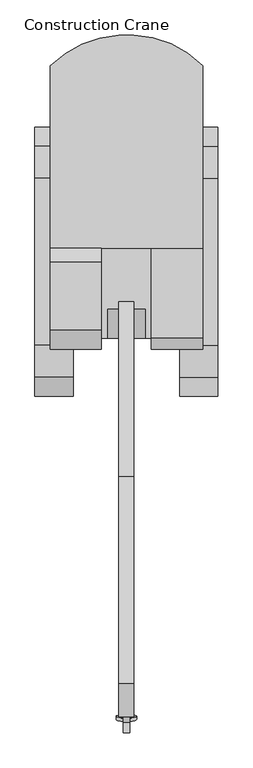
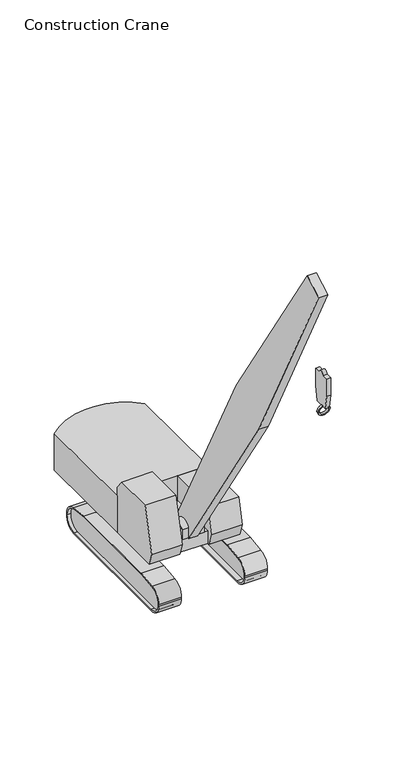
"""IFC4 building model written with IfcOpenShell, lengths in millimetres: geographic element geometry, Construction Crane : 50' @ 60 deg."""

from ifc_helpers import new_model, si_unit, point, frame, frame_2d, origin, place, context, project, spatial, polyline, circle_curve, trimmed, segment, composite_curve, outline, extrude, source, transform, mapped, element, save


def construction_crane_787d4a5c(model_context):
    return source(origin(), model_context, "Body", "SweptSolid", [
        extrude(outline(composite_curve([segment(polyline([(-4575.608491, 934.26875), (-1239.0684321, 934.26875), (-625.3121051, 856.1386871)]), True, "CONTINUOUS"), segment(trimmed(circle_curve(frame_2d((-676.8331731, 453.3411993)), 406.0791014), [point((-625.3121051, 856.1386871))], [point((-270.7700765, 456.946505))], False, "CARTESIAN"), True, "CONTINUOUS"), segment(trimmed(circle_curve(frame_2d((-676.7161092, 456.946505)), 405.9460328), [point((-270.7700765, 456.946505))], [point((-676.7161092, 51.0004722))], False, "CARTESIAN"), True, "CONTINUOUS"), segment(polyline([(-676.7161092, 51.0004722), (-5143.9371049, 51.0004722)]), True, "CONTINUOUS"), segment(trimmed(circle_curve(frame_2d((-5143.9371049, 451.7022639)), 400.7017917), [point((-5143.9371049, 51.0004722))], [point((-5544.6388966, 451.7022639))], False, "CARTESIAN"), True, "CONTINUOUS"), segment(trimmed(circle_curve(frame_2d((-5137.6945084, 451.7710081)), 406.944394), [point((-5544.6388966, 451.7022639))], [point((-5189.1160735, 855.4535101))], False, "CARTESIAN"), True, "CONTINUOUS"), segment(polyline([(-5189.1160735, 855.4535101), (-4575.608491, 934.26875)]), True, "CONTINUOUS")], self_intersect=False)), frame((-4426.6809216, 0.0, 0.0), z_axis=(1.0, 0.0, 0.0), x_axis=(0.0, 1.0, 0.0)), (0.0, 0.0, 1.0), 464.6393791),
        extrude(outline(composite_curve([segment(polyline([(-651.6384615, 0.0), (-5163.0384615, 0.0)]), True, "CONTINUOUS"), segment(trimmed(circle_curve(frame_2d((-5163.0384615, 431.8)), 431.8), [point((-5163.0384615, 0.0))], [point((-5594.8384615, 431.8))], False, "CARTESIAN"), True, "CONTINUOUS"), segment(polyline([(-5594.8384615, 431.8), (-5594.8384615, 475.1036968)]), True, "CONTINUOUS"), segment(trimmed(circle_curve(frame_2d((-5163.0384615, 475.1036968)), 431.8), [point((-5594.8384615, 475.1036968))], [point((-5217.7268735, 903.4264928))], False, "CARTESIAN"), True, "CONTINUOUS"), segment(polyline([(-5217.7268735, 903.4264928), (-4578.8384615, 985.06875), (-1235.8384615, 985.06875), (-596.9500496, 903.4264928)]), True, "CONTINUOUS"), segment(trimmed(circle_curve(frame_2d((-651.6384615, 475.1036968)), 431.8), [point((-596.9500496, 903.4264928))], [point((-219.8384615, 475.1036968))], False, "CARTESIAN"), True, "CONTINUOUS"), segment(polyline([(-219.8384615, 475.1036968), (-219.8384615, 431.8)]), True, "CONTINUOUS"), segment(trimmed(circle_curve(frame_2d((-651.6384615, 431.8)), 431.8), [point((-219.8384615, 431.8))], [point((-651.6384615, 0.0))], False, "CARTESIAN"), True, "CONTINUOUS")], self_intersect=False), holes=[composite_curve([segment(polyline([(-4575.608491, 934.26875), (-5189.1160735, 855.3847601)]), True, "CONTINUOUS"), segment(trimmed(circle_curve(frame_2d((-5137.6945084, 451.7022639)), 406.9443882), [point((-5189.1160735, 855.3847601))], [point((-5544.6388966, 451.7022639))], True, "CARTESIAN"), True, "CONTINUOUS"), segment(trimmed(circle_curve(frame_2d((-5143.9371049, 451.7022639)), 400.7017917), [point((-5544.6388966, 451.7022639))], [point((-5143.9371049, 51.0004722))], True, "CARTESIAN"), True, "CONTINUOUS"), segment(polyline([(-5143.9371049, 51.0004722), (-676.7161092, 51.0004722)]), True, "CONTINUOUS"), segment(trimmed(circle_curve(frame_2d((-676.7161092, 456.946505)), 405.9460328), [point((-676.7161092, 51.0004722))], [point((-270.7700765, 456.946505))], True, "CARTESIAN"), True, "CONTINUOUS"), segment(trimmed(circle_curve(frame_2d((-676.8331731, 453.2718224)), 406.0797233), [point((-270.7700765, 456.946505))], [point((-625.3121051, 856.0699371))], True, "CARTESIAN"), True, "CONTINUOUS"), segment(polyline([(-625.3121051, 856.0699371), (-1239.0684321, 934.26875), (-4575.608491, 934.26875)]), True, "CONTINUOUS")], self_intersect=False)]), frame((-4612.32123, 0.0, 0.0), z_axis=(1.0, 0.0, 0.0), x_axis=(0.0, 1.0, 0.0)), (0.0, 0.0, 1.0), 762.0),
        extrude(outline(composite_curve([segment(polyline([(-4575.608491, 934.26875), (-1239.0684321, 934.26875), (-625.3121051, 856.1386871)]), True, "CONTINUOUS"), segment(trimmed(circle_curve(frame_2d((-676.8331731, 453.3411993)), 406.0791014), [point((-625.3121051, 856.1386871))], [point((-270.7700765, 456.946505))], False, "CARTESIAN"), True, "CONTINUOUS"), segment(trimmed(circle_curve(frame_2d((-676.7161092, 456.946505)), 405.9460328), [point((-270.7700765, 456.946505))], [point((-676.7161092, 51.0004722))], False, "CARTESIAN"), True, "CONTINUOUS"), segment(polyline([(-676.7161092, 51.0004722), (-5143.9005487, 51.0004722)]), True, "CONTINUOUS"), segment(trimmed(circle_curve(frame_2d((-5143.9005487, 451.7388201)), 400.738348), [point((-5143.9005487, 51.0004722))], [point((-5544.6388966, 451.7388201))], False, "CARTESIAN"), True, "CONTINUOUS"), segment(trimmed(circle_curve(frame_2d((-5137.6579522, 451.7388201)), 406.9809445), [point((-5544.6388966, 451.7388201))], [point((-5189.1160735, 855.4535101))], False, "CARTESIAN"), True, "CONTINUOUS"), segment(polyline([(-5189.1160735, 855.4535101), (-4575.608491, 934.26875)]), True, "CONTINUOUS")], self_intersect=False)), frame((-7396.2009175, 0.0, 0.0), z_axis=(1.0, 0.0, 0.0), x_axis=(0.0, 1.0, 0.0)), (0.0, 0.0, 1.0), 464.6393791),
        extrude(outline(composite_curve([segment(polyline([(-3855.5873985, 1944.8065119), (-3855.5873985, 1589.2065119), (-4435.4967838, 1589.2065119), (-4435.4967838, 1944.8065119)]), True, "CONTINUOUS"), segment(trimmed(circle_curve(frame_2d((-4145.5420911, 1746.7297499)), 351.15257), [point((-4435.4967838, 1944.8065119))], [point((-3855.5873985, 1944.8065119))], False, "CARTESIAN"), True, "CONTINUOUS")], self_intersect=False)), frame((-6056.08998, 0.0, 0.0), z_axis=(1.0, 0.0, 0.0), x_axis=(0.0, 1.0, 0.0)), (0.0, 0.0, 1.0), 755.1034902),
        extrude(outline(polyline([(-5179.12123, -2642.3288049), (-5179.12123, -4433.7384615), (-6179.12123, -4433.7384615), (-6179.12123, -2642.3288049), (-5179.12123, -2642.3288049)])), frame((0.0, 0.0, 1155.0), z_axis=(0.0, 0.0, 1.0), x_axis=(1.0, 0.0, 0.0)), (0.0, 0.0, 1.0), 434.1377619),
        extrude(outline(composite_curve([segment(polyline([(-651.6384615, 0.0), (-5163.0384615, 0.0)]), True, "CONTINUOUS"), segment(trimmed(circle_curve(frame_2d((-5163.0384615, 431.8)), 431.8), [point((-5163.0384615, 0.0))], [point((-5594.8384615, 431.8))], False, "CARTESIAN"), True, "CONTINUOUS"), segment(polyline([(-5594.8384615, 431.8), (-5594.8384615, 475.1036968)]), True, "CONTINUOUS"), segment(trimmed(circle_curve(frame_2d((-5163.0384615, 475.1036968)), 431.8), [point((-5594.8384615, 475.1036968))], [point((-5217.7268735, 903.4264928))], False, "CARTESIAN"), True, "CONTINUOUS"), segment(polyline([(-5217.7268735, 903.4264928), (-4578.8384615, 985.06875), (-1235.8384615, 985.06875), (-596.9500496, 903.4264928)]), True, "CONTINUOUS"), segment(trimmed(circle_curve(frame_2d((-651.6384615, 475.1036968)), 431.8), [point((-596.9500496, 903.4264928))], [point((-219.8384615, 475.1036968))], False, "CARTESIAN"), True, "CONTINUOUS"), segment(polyline([(-219.8384615, 475.1036968), (-219.8384615, 431.8)]), True, "CONTINUOUS"), segment(trimmed(circle_curve(frame_2d((-651.6384615, 431.8)), 431.8), [point((-219.8384615, 431.8))], [point((-651.6384615, 0.0))], False, "CARTESIAN"), True, "CONTINUOUS")], self_intersect=False), holes=[composite_curve([segment(polyline([(-4575.608491, 934.26875), (-5189.1160735, 855.3847601)]), True, "CONTINUOUS"), segment(trimmed(circle_curve(frame_2d((-5137.6945084, 451.7022639)), 406.9443882), [point((-5189.1160735, 855.3847601))], [point((-5544.6388966, 451.7022639))], True, "CARTESIAN"), True, "CONTINUOUS"), segment(trimmed(circle_curve(frame_2d((-5143.9371049, 451.7022639)), 400.7017917), [point((-5544.6388966, 451.7022639))], [point((-5143.9371049, 51.0004722))], True, "CARTESIAN"), True, "CONTINUOUS"), segment(polyline([(-5143.9371049, 51.0004722), (-676.7161092, 51.0004722)]), True, "CONTINUOUS"), segment(trimmed(circle_curve(frame_2d((-676.7161092, 456.946505)), 405.9460328), [point((-676.7161092, 51.0004722))], [point((-270.7700765, 456.946505))], True, "CARTESIAN"), True, "CONTINUOUS"), segment(trimmed(circle_curve(frame_2d((-676.8331731, 453.2718224)), 406.0797233), [point((-270.7700765, 456.946505))], [point((-625.3121051, 856.0699371))], True, "CARTESIAN"), True, "CONTINUOUS"), segment(polyline([(-625.3121051, 856.0699371), (-1239.0684321, 934.26875), (-4575.608491, 934.26875)]), True, "CONTINUOUS")], self_intersect=False)]), frame((-7507.92123, 0.0, 0.0), z_axis=(1.0, 0.0, 0.0), x_axis=(0.0, 1.0, 0.0)), (0.0, 0.0, 1.0), 762.0),
        extrude(outline(composite_curve([segment(polyline([(-7203.12123, -2642.3288049), (-7203.12123, 1015.2711951)]), True, "CONTINUOUS"), segment(trimmed(circle_curve(frame_2d((-5666.4440826, -594.4023865)), 2225.4046136), [point((-7203.12123, 1015.2711951))], [point((-5831.52123, 1624.8711951))], False, "CARTESIAN"), True, "CONTINUOUS"), segment(polyline([(-5831.52123, 1624.8711951), (-5526.72123, 1624.8711951)]), True, "CONTINUOUS"), segment(trimmed(circle_curve(frame_2d((-5627.7327269, -450.2546729)), 2077.5828962), [point((-5526.72123, 1624.8711951))], [point((-4155.12123, 1015.2711951))], False, "CARTESIAN"), True, "CONTINUOUS"), segment(polyline([(-4155.12123, 1015.2711951), (-4155.12123, -2642.3288049), (-7203.12123, -2642.3288049)]), True, "CONTINUOUS")], self_intersect=False)), frame((0.0, 0.0, 1155.0), z_axis=(0.0, 0.0, 1.0), x_axis=(1.0, 0.0, 0.0)), (0.0, 0.0, 1.0), 1300.06875),
        extrude(outline(polyline([(-2642.3288049, 1155.06875), (-4509.1429639, 1155.06875), (-4662.3384615, 1584.1295061), (-4443.5105446, 2455.06875), (-2642.3288049, 2455.06875), (-2642.3288049, 1155.06875)])), frame((-5179.12123, 0.0, 0.0), z_axis=(1.0, 0.0, 0.0), x_axis=(0.0, 1.0, 0.0)), (0.0, 0.0, 1.0), 1024.0),
        extrude(outline(polyline([(-2642.3288049, 2759.86875), (-2642.3288049, 2455.06875), (-2642.3288049, 1155.06875), (-4509.1429639, 1155.06875), (-4662.3384615, 1584.1295061), (-4278.9384615, 3110.06875), (-2907.3384615, 3110.06875), (-2642.3288049, 2759.86875)])), frame((-7203.12123, 0.0, 0.0), z_axis=(1.0, 0.0, 0.0), x_axis=(0.0, 1.0, 0.0)), (0.0, 0.0, 1.0), 1024.0),
        extrude(outline(polyline([(-7211.0827225, 8686.8431812), (-3709.0413561, 1909.9296043), (-4412.9468043, 1503.5296043), (-8530.9054378, 7924.8431812), (-12010.949759, 14714.456758), (-11351.0384013, 15095.456758), (-7211.0827225, 8686.8431812)])), frame((-5831.52123, 0.0, 0.0), z_axis=(1.0, 0.0, 0.0), x_axis=(0.0, 1.0, 0.0)), (0.0, 0.0, 1.0), 304.8),
        extrude(outline(composite_curve([segment(trimmed(circle_curve(frame_2d((0.0, -203.2)), 203.2), [point((0.0, -406.4))], [point((0.0, 0.0))], False, "CARTESIAN"), True, "CONTINUOUS"), segment(trimmed(circle_curve(frame_2d((0.0, -203.2)), 203.2), [point((0.0, 0.0))], [point((0.0, -406.4))], False, "CARTESIAN"), True, "CONTINUOUS")], self_intersect=False), holes=[composite_curve([segment(trimmed(circle_curve(frame_2d((0.0, -203.2)), 152.4), [point((0.0, -355.6))], [point((0.0, -50.8))], True, "CARTESIAN"), True, "CONTINUOUS"), segment(trimmed(circle_curve(frame_2d((0.0, -203.2)), 152.4), [point((0.0, -50.8))], [point((0.0, -355.6))], True, "CARTESIAN"), True, "CONTINUOUS")], self_intersect=False)]), frame((-5475.92123, -12062.2674955, 10688.4197702), z_axis=(0.0, 0.9808984463456898, 0.1945205335089642), x_axis=(0.0, -0.1945205335089642, 0.9808984463456898)), (0.0, 0.0, 1.0), 62.999),
        extrude(outline(composite_curve([segment(polyline([(-11903.8512674, 11971.256758), (-11687.9512674, 11971.256758), (-11687.9512674, 11361.656758), (-11776.1645417, 10861.3744195), (-12234.7379931, 10861.3744195), (-12333.9482506, 11361.656758), (-12333.9482506, 11971.256758), (-12118.0482506, 11971.256758)]), True, "CONTINUOUS"), segment(trimmed(circle_curve(frame_2d((-12010.949759, 11971.256758)), 107.0984916), [point((-12118.0482506, 11971.256758))], [point((-11903.8512674, 11971.256758))], False, "CARTESIAN"), True, "CONTINUOUS")], self_intersect=False)), frame((-5743.7360332, 0.0, 0.0), z_axis=(1.0, 0.0, 0.0), x_axis=(0.0, 1.0, 0.0)), (0.0, 0.0, 1.0), 133.1095203),
    ])


if __name__ == "__main__":
    model = new_model("IFC4")
    model_context = context("Model", 3, world=origin())
    ifc_project = project(units=[si_unit("LENGTHUNIT", "METRE", prefix="MILLI")], contexts=[model_context])
    site = spatial("IfcSite", under=ifc_project)
    building = spatial("IfcBuilding", under=site)
    placement = place(None, origin())
    construction_crane_shape = construction_crane_787d4a5c(model_context)
    element("IfcGeographicElement", 1, ObjectType="Construction Crane : 50' @ 60 deg", at=placement, inside=building, context=model_context, shape_type="MappedRepresentation", body=[
        mapped(construction_crane_shape, transform((0.0, 0.0, 0.0), x_axis=(1.0, 0.0, 0.0), y_axis=(0.0, 1.0, 0.0), z_axis=(0.0, 0.0, 1.0))),
    ])
    save(model, "model.ifc")

# Revit data of these elements
# Type "Construction Crane : 50' @ 60 deg"
#   Boom Angle = 60.00°
#   Boom Half = 25' - 0"
#   Boom Length = 50' - 0"
#   Cab Width = 10' - 0"
#   Counter Weight = 14' - 0"
#   Hook = 30.00°
#   Turning Radius = 15' - 0"
#   Width = 12' - 0"
# Element 1 (IfcGeographicElement, "Construction Crane : 50' @ 60 deg")
#   Materials on its faces: "Metal, Paint Finish, White, Matte", "Plastic, Opaque Black", "Steel"
# Materials
#   "Metal, Paint Finish, White, Matte": class "Metal", colour RGB 247 247 239, transparency 0, Description = "Paint finished steel", Cost = 0
#   "Plastic, Opaque Black": class "Plastic", colour RGB 0 0 0, transparency 0, Description = "Plastic, generic, opaque black", Cost = 0
#   "Steel": class "Metal", colour RGB 128 128 128, transparency 0, Description = "Steel, mill finish", Cost = 0
